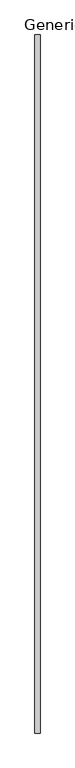
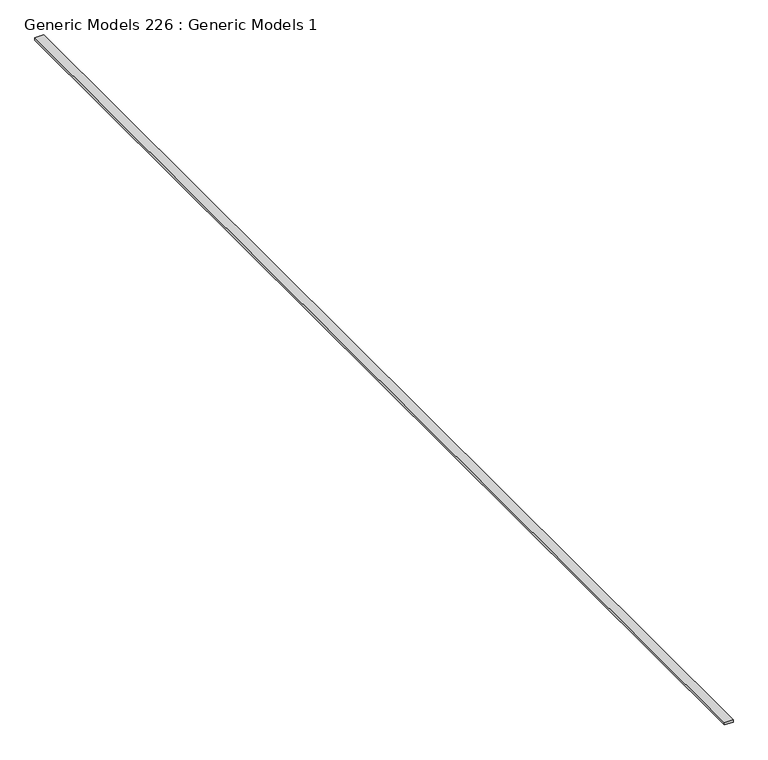
"""IFC4 building model written with IfcOpenShell, lengths in millimetres: proxy geometry, Generic Models 226 : Generic Models 1."""

from ifc_helpers import new_model, si_unit, frame, origin, place, context, project, spatial, polyline, outline, extrude, source, transform, mapped, element, save


def generic_models_226_generic_models_1_2b807524(model_context):
    return source(origin(), model_context, "Body", "SweptSolid", [
        extrude(outline(polyline([(-73110.2594513, 44054.5282881), (-72970.5594513, 44054.5282881), (-72970.5594513, 25004.5282881), (-73110.2594513, 25004.5282881), (-73110.2594513, 44054.5282881)])), frame((0.0, 0.0, 124623.1032403), z_axis=(0.0, 0.0, 1.0), x_axis=(1.0, 0.0, 0.0)), (0.0, 0.0, 1.0), 38.1),
    ])


if __name__ == "__main__":
    model = new_model("IFC4")
    model_context = context("Model", 3, world=origin())
    ifc_project = project(units=[si_unit("LENGTHUNIT", "METRE", prefix="MILLI")], contexts=[model_context])
    site = spatial("IfcSite", under=ifc_project)
    building = spatial("IfcBuilding", under=site)
    placement = place(None, origin())
    generic_models_226_generic_models_1_shape = generic_models_226_generic_models_1_2b807524(model_context)
    element("IfcBuildingElementProxy", 1, Name="Generic Models 226 : Generic Models 1", ObjectType="Generic Models 226 : Generic Models 1", at=placement, inside=building, context=model_context, shape_type="MappedRepresentation", body=[
        mapped(generic_models_226_generic_models_1_shape, transform((0.0, 0.0, 0.0), x_axis=(1.0, 0.0, 0.0), y_axis=(0.0, 1.0, 0.0), z_axis=(0.0, 0.0, 1.0))),
    ])
    save(model, "model.ifc")

# Revit data of these elements
# Element 1 (IfcBuildingElementProxy, "Generic Models 226 : Generic Models 1")
#   Materials on its faces: "_2X BLOCKING AS REQUIRED"
# Materials
#   "_2X BLOCKING AS REQUIRED": class "Generic", colour RGB 177 130 114, transparency 0, Cost = 0
